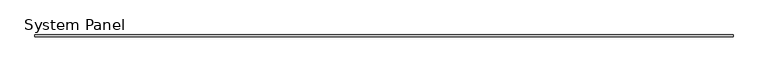
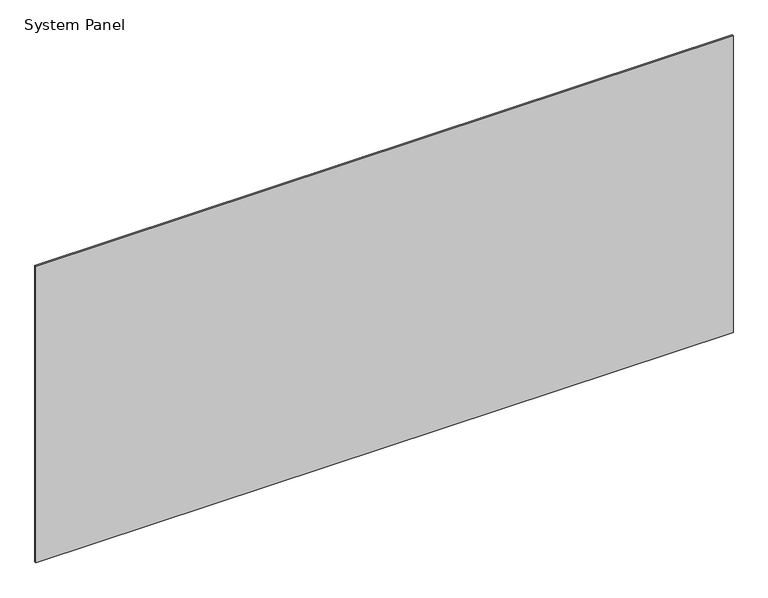
"""IFC4 building model written with IfcOpenShell, lengths in millimetres: plate geometry, System Panel : 로이복층유리_16."""

from ifc_helpers import new_model, si_unit, frame, origin, place, context, project, spatial, polyline, outline, extrude, source, transform, mapped, element, save


def system_panel_2e5c4234(model_context):
    return source(origin(), model_context, "Body", "SweptSolid", [
        extrude(outline(polyline([(0.0, -3284.5), (0.0, 3284.5), (2177.5, 3284.5), (2955.0, 3284.5), (2955.0, -3284.5), (2177.5, -3284.5), (0.0, -3284.5)])), frame((0.0, -8.0, 0.0), z_axis=(0.0, 1.0, 0.0), x_axis=(0.0, 0.0, 1.0)), (0.0, 0.0, 1.0), 16.0),
    ])


if __name__ == "__main__":
    model = new_model("IFC4")
    model_context = context("Model", 3, world=origin())
    ifc_project = project(units=[si_unit("LENGTHUNIT", "METRE", prefix="MILLI")], contexts=[model_context])
    site = spatial("IfcSite", under=ifc_project)
    building = spatial("IfcBuilding", under=site)
    placement = place(None, origin())
    system_panel_shape = system_panel_2e5c4234(model_context)
    element("IfcPlate", 1, ObjectType="System Panel : 로이복층유리_16", at=placement, inside=building, context=model_context, shape_type="MappedRepresentation", body=[
        mapped(system_panel_shape, transform((0.0, 0.0, 0.0), x_axis=(1.0, 0.0, 0.0), y_axis=(0.0, 1.0, 0.0), z_axis=(0.0, 0.0, 1.0))),
    ])
    save(model, "model.ifc")

# Revit data of these elements
# Element 1 (IfcPlate, "System Panel : 로이복층유리_16")
#   Materials on its faces: "00_Glass_Glass"
# Materials
#   "00_Glass_Glass": class "Glass", colour RGB 218 227 224, transparency 0.85, Description = "Glass", Cost = 0, Image = none
